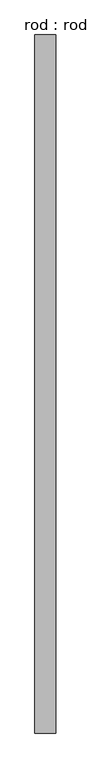
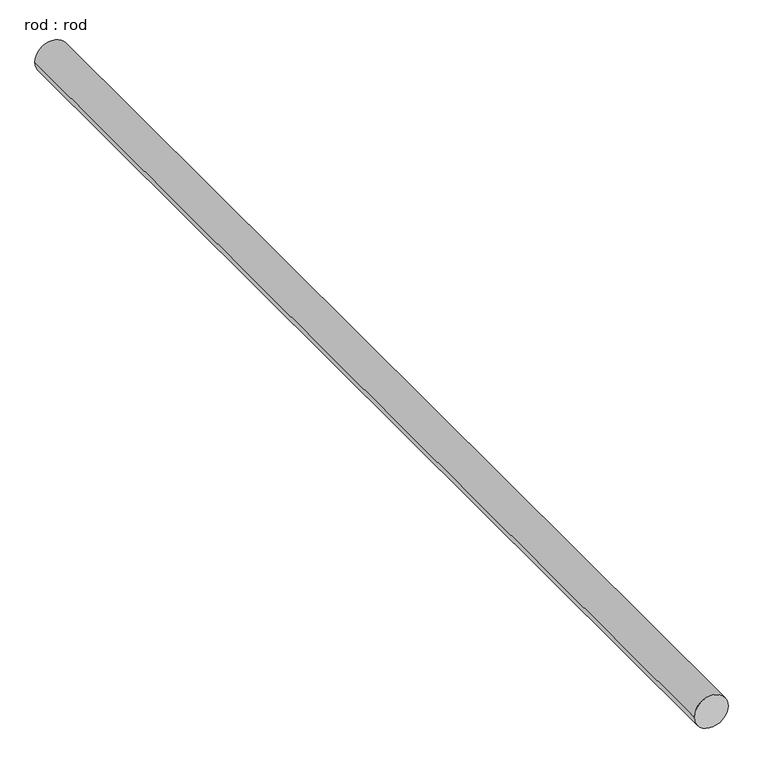
"""IFC4 building model written with IfcOpenShell, lengths in millimetres: proxy geometry, rod : rod."""

from ifc_helpers import new_model, si_unit, point, frame, frame_2d, origin, place, context, project, spatial, circle_curve, trimmed, segment, composite_curve, outline, extrude, source, transform, mapped, element, save


def rod_rod_15d67a72(model_context):
    return source(origin(), model_context, "Body", "SweptSolid", [
        extrude(outline(composite_curve([segment(trimmed(circle_curve(frame_2d((0.0108462, 0.0)), 200.0), [point((0.0108462, 200.0))], [point((0.0108462, -200.0))], False, "CARTESIAN"), True, "CONTINUOUS"), segment(trimmed(circle_curve(frame_2d((0.0108462, 0.0)), 200.0), [point((0.0108462, -200.0))], [point((0.0108462, 200.0))], False, "CARTESIAN"), True, "CONTINUOUS")], self_intersect=False)), frame((0.0, -2657.2713847, 0.0), z_axis=(0.0, 1.0, 0.0), x_axis=(0.0, 0.0, 1.0)), (0.0, 0.0, 1.0), 13500.0),
    ])


if __name__ == "__main__":
    model = new_model("IFC4")
    model_context = context("Model", 3, world=origin())
    ifc_project = project(units=[si_unit("LENGTHUNIT", "METRE", prefix="MILLI")], contexts=[model_context])
    site = spatial("IfcSite", under=ifc_project)
    building = spatial("IfcBuilding", under=site)
    placement = place(None, origin())
    rod_rod_shape = rod_rod_15d67a72(model_context)
    element("IfcBuildingElementProxy", 1, Name="rod : rod", ObjectType="rod : rod", at=placement, inside=building, context=model_context, shape_type="MappedRepresentation", body=[
        mapped(rod_rod_shape, transform((0.0, 0.0, 0.0), x_axis=(1.0, 0.0, 0.0), y_axis=(0.0, 1.0, 0.0), z_axis=(0.0, 0.0, 1.0))),
    ])
    save(model, "model.ifc")

# Revit data of these elements
# Type "rod : rod"
#   Default Elevation = 0
